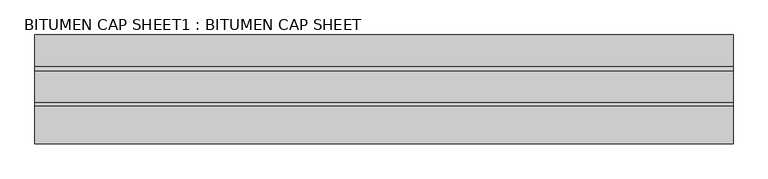
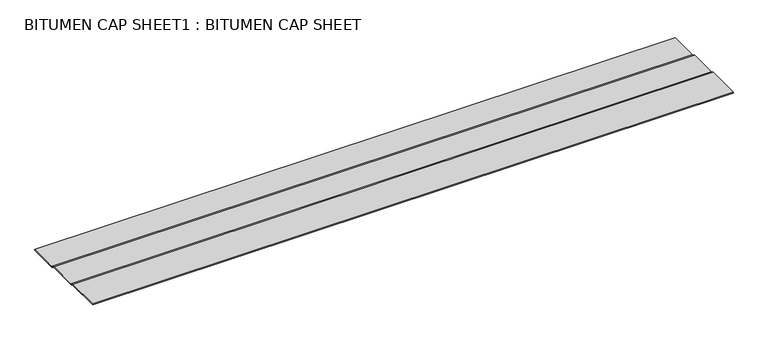
"""IFC4 building model written with IfcOpenShell, lengths in millimetres: proxy geometry, BITUMEN CAP SHEET1 : BITUMEN CAP SHEET."""

from ifc_helpers import new_model, si_unit, frame, origin, place, context, project, spatial, polyline, outline, extrude, source, transform, mapped, element, save


def bitumen_cap_sheet1_bitumen_cap_sheet_a55ad838(model_context):
    return source(origin(), model_context, "Body", "SweptSolid", [
        extrude(outline(polyline([(-5237.2758356, 40238.7580714), (-5329.4404972, 40238.7580714), (-5341.9053158, 40244.0440809), (-5432.619472, 40244.0440809), (-5442.3358585, 40248.3766459), (-5549.5470696, 40248.3766459), (-5549.5470696, 40251.5518755), (-5441.660573, 40251.5518755), (-5431.9436715, 40247.2190809), (-5341.2599159, 40247.2190809), (-5328.7950972, 40241.9330714), (-5237.2758356, 40241.9330714), (-5237.2758356, 40238.7580714)])), frame((12382.7678845, 0.0, 0.0), z_axis=(1.0, 0.0, 0.0), x_axis=(0.0, 1.0, 0.0)), (0.0, 0.0, 1.0), 2000.25),
    ])


if __name__ == "__main__":
    model = new_model("IFC4")
    model_context = context("Model", 3, world=origin())
    ifc_project = project(units=[si_unit("LENGTHUNIT", "METRE", prefix="MILLI")], contexts=[model_context])
    site = spatial("IfcSite", under=ifc_project)
    building = spatial("IfcBuilding", under=site)
    placement = place(None, origin())
    bitumen_cap_sheet1_bitumen_cap_sheet_shape = bitumen_cap_sheet1_bitumen_cap_sheet_a55ad838(model_context)
    element("IfcBuildingElementProxy", 1, Name="BITUMEN CAP SHEET1 : BITUMEN CAP SHEET", ObjectType="BITUMEN CAP SHEET1 : BITUMEN CAP SHEET", at=placement, inside=building, context=model_context, shape_type="MappedRepresentation", body=[
        mapped(bitumen_cap_sheet1_bitumen_cap_sheet_shape, transform((0.0, 0.0, 0.0), x_axis=(1.0, 0.0, 0.0), y_axis=(0.0, 1.0, 0.0), z_axis=(0.0, 0.0, 1.0))),
    ])
    save(model, "model.ifc")

# Revit data of these elements
# Type "BITUMEN CAP SHEET1 : BITUMEN CAP SHEET"
#   NameOverride = "BITUMEN CAP SHEET"
# Element 1 (IfcBuildingElementProxy, "BITUMEN CAP SHEET1 : BITUMEN CAP SHEET")
#   Materials on its faces: "MODIFIED BITUMEN GRANULE SURFACED CAP SHEET"
# Materials
#   "MODIFIED BITUMEN GRANULE SURFACED CAP SHEET": class "Unassigned", colour RGB 85 85 127, transparency 0
